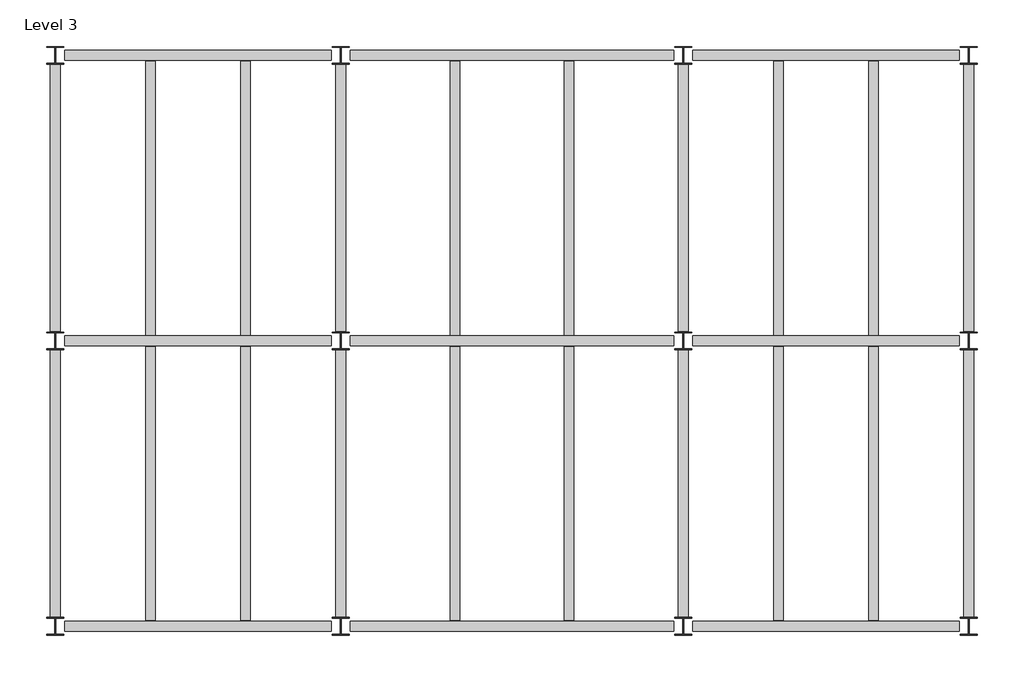
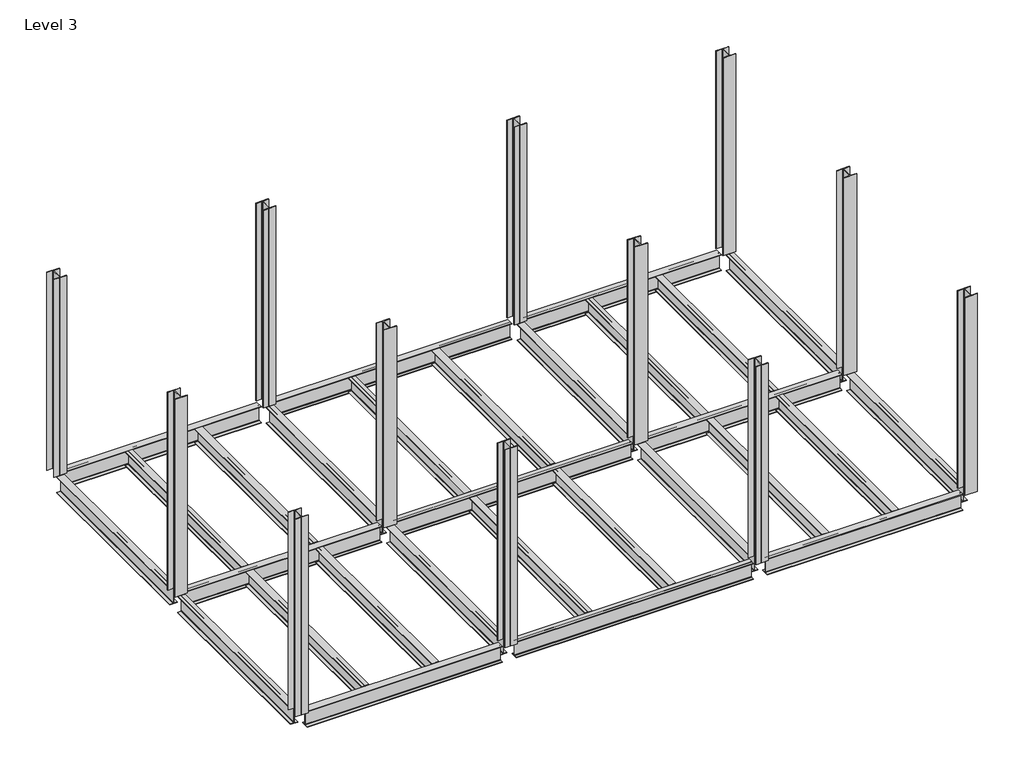
# One storey: 29 beams, 12 columns.
"""IFC4 building model written with IfcOpenShell, lengths in millimetres."""

import ifcopenshell
import ifcopenshell.guid

model = None  # the IFC model being written
_history = None  # IfcOwnerHistory: only IFC2X3 demands one
_inside = {}  # id of a spatial element -> (the spatial element, [elements in it])
_under = {}  # id of a project, library or spatial element -> (it, [spatial elements below it])
_declared = {}  # id of a project -> (the project, [libraries it declares])
_typed = {}  # id of a type object -> (the type object, [elements of that type])
_made_of = {}  # id of a material, layer set ... -> (it, [elements and type objects made of it])


def new_model(schema):
    """Start an empty IFC model of exactly this schema.

    Asked for "IFC4X3", IfcOpenShell would pick the latest addendum, in which some entities
    have other attributes; the version numbers below select the first issue.
    IFC2X3 requires an IfcOwnerHistory on every rooted entity: one is made here for all.
    """
    global model, _history
    if schema == "IFC4X3":
        model = ifcopenshell.file(schema_version=(4, 3, 0, 0))
    else:
        model = ifcopenshell.file(schema=schema)
    _inside.clear()
    _under.clear()
    _declared.clear()
    _typed.clear()
    _made_of.clear()
    _history = None
    if model.schema == "IFC2X3":
        org = make("IfcOrganization", Name="unknown")
        user = make(
            "IfcPersonAndOrganization",
            ThePerson=make("IfcPerson", FamilyName="unknown"),
            TheOrganization=org,
        )
        app = make(
            "IfcApplication",
            ApplicationDeveloper=org,
            Version="unknown",
            ApplicationFullName="unknown",
            ApplicationIdentifier="unknown",
        )
        _history = make(
            "IfcOwnerHistory",
            OwningUser=user,
            OwningApplication=app,
            ChangeAction="ADDED",
            CreationDate=0,
        )
    return model


def make(cls, **values):
    """One entity of the class cls with the attributes given. An attribute that is None is left unset."""
    return model.create_entity(
        cls, **{name: value for name, value in values.items() if value is not None}
    )


def rooted(cls, **values):
    """An entity with a GlobalId (a new one), such as an element, a storey or a relation."""
    return make(cls, GlobalId=ifcopenshell.guid.new(), OwnerHistory=_history, **values)


def si_unit(unit_type, name, prefix=None):
    """IfcSIUnit, for example si_unit("LENGTHUNIT", "METRE", prefix="MILLI")."""
    return make("IfcSIUnit", UnitType=unit_type, Prefix=prefix, Name=name)


def assignment(units):
    """IfcUnitAssignment: the units of a project."""
    return None if units is None else make("IfcUnitAssignment", Units=units)


def point(xyz):
    """IfcCartesianPoint."""
    return None if xyz is None else make("IfcCartesianPoint", Coordinates=xyz)


def direction(xyz):
    """IfcDirection."""
    return None if xyz is None else make("IfcDirection", DirectionRatios=xyz)


def frame(location, z_axis=None, x_axis=None):
    """IfcAxis2Placement3D, a coordinate frame: its origin and axes. An axis left out is left unset."""
    return make(
        "IfcAxis2Placement3D",
        Location=point(location),
        Axis=direction(z_axis),
        RefDirection=direction(x_axis),
    )


def frame_2d(location, x_axis=None):
    """IfcAxis2Placement2D, a coordinate frame in the plane: its origin and x axis."""
    return make(
        "IfcAxis2Placement2D", Location=point(location), RefDirection=direction(x_axis)
    )


def origin():
    """The frame at (0, 0, 0) with its axes left unset."""
    return frame((0.0, 0.0, 0.0))


def place(relative_to, where):
    """IfcLocalPlacement: puts the frame where relative to a parent placement (None: the world)."""
    return make(
        "IfcLocalPlacement", PlacementRelTo=relative_to, RelativePlacement=where
    )


def context(
    kind, dimensions, precision=None, world=None, true_north=None, identifier=None
):
    """IfcGeometricRepresentationContext, for example the 3D "Model" context."""
    return make(
        "IfcGeometricRepresentationContext",
        ContextIdentifier=identifier,
        ContextType=kind,
        CoordinateSpaceDimension=dimensions,
        Precision=precision,
        WorldCoordinateSystem=world,
        TrueNorth=true_north,
    )


def project(units=None, contexts=None):
    """IfcProject with its units and contexts."""
    return rooted(
        "IfcProject",
        Name="project",
        RepresentationContexts=contexts,
        UnitsInContext=assignment(units),
    )


def spatial(cls, under=None, at=None, **own):
    """A site, building, storey or space (cls), placed at a placement, below another one or the project."""
    s = rooted(cls, ObjectPlacement=at, **own)
    if under is not None:
        _under.setdefault(under.id(), (under, []))[1].append(s)
    return s


def polyline(points):
    """IfcPolyline through the points."""
    return make("IfcPolyline", Points=[point(p) for p in points])


def circle_curve(where, radius):
    """IfcCircle in the frame where."""
    return make("IfcCircle", Position=where, Radius=radius)


def trimmed(basis, trim1, trim2, sense, master):
    """IfcTrimmedCurve: the piece of a basis curve between two trims."""
    return make(
        "IfcTrimmedCurve",
        BasisCurve=basis,
        Trim1=trim1,
        Trim2=trim2,
        SenseAgreement=sense,
        MasterRepresentation=master,
    )


def segment(curve, same_sense, transition):
    """IfcCompositeCurveSegment."""
    return make(
        "IfcCompositeCurveSegment",
        Transition=transition,
        SameSense=same_sense,
        ParentCurve=curve,
    )


def composite_curve(segments, self_intersect=None):
    """IfcCompositeCurve: segments joined end to end."""
    return make("IfcCompositeCurve", Segments=segments, SelfIntersect=self_intersect)


def outline(outer, holes=None, kind="AREA"):
    """IfcArbitraryClosedProfileDef: a profile drawn as a closed curve; with holes, ...WithVoids."""
    if holes is None:
        return make("IfcArbitraryClosedProfileDef", ProfileType=kind, OuterCurve=outer)
    return make(
        "IfcArbitraryProfileDefWithVoids",
        ProfileType=kind,
        OuterCurve=outer,
        InnerCurves=holes,
    )


def extrude(swept, where, along, depth):
    """IfcExtrudedAreaSolid: the profile swept, set in the frame where, extruded along a direction by depth."""
    return make(
        "IfcExtrudedAreaSolid",
        SweptArea=swept,
        Position=where,
        ExtrudedDirection=direction(along),
        Depth=depth,
    )


def shape(context_of_items, identifier, shape_type, items):
    """IfcShapeRepresentation: the items that make up one representation, for example the "Body"."""
    return make(
        "IfcShapeRepresentation",
        ContextOfItems=context_of_items,
        RepresentationIdentifier=identifier,
        RepresentationType=shape_type,
        Items=items,
    )


def source(mapping_origin, context_of_items, identifier, shape_type, items):
    """IfcRepresentationMap: a shape defined once, which mapped items show again and again."""
    return make(
        "IfcRepresentationMap",
        MappingOrigin=mapping_origin,
        MappedRepresentation=shape(context_of_items, identifier, shape_type, items),
    )


def transform(
    local_origin,
    x_axis=None,
    y_axis=None,
    z_axis=None,
    scale=None,
    scale2=None,
    scale3=None,
    uniform=True,
):
    """IfcCartesianTransformationOperator3D, or its non-uniform kind. x_axis, y_axis, z_axis: its Axis1, 2, 3."""
    if uniform:
        return make(
            "IfcCartesianTransformationOperator3D",
            Axis1=direction(x_axis),
            Axis2=direction(y_axis),
            LocalOrigin=point(local_origin),
            Scale=scale,
            Axis3=direction(z_axis),
        )
    return make(
        "IfcCartesianTransformationOperator3DnonUniform",
        Axis1=direction(x_axis),
        Axis2=direction(y_axis),
        LocalOrigin=point(local_origin),
        Scale=scale,
        Axis3=direction(z_axis),
        Scale2=scale2,
        Scale3=scale3,
    )


def mapped(mapping_source, mapping_target):
    """IfcMappedItem: shows the shape of a source again, moved by a transform."""
    return make(
        "IfcMappedItem", MappingSource=mapping_source, MappingTarget=mapping_target
    )


def made_of(thing, what):
    """Note that an element or type object is made of a material, layer set ...; save() writes the relation."""
    if what is not None:
        _made_of.setdefault(what.id(), (what, []))[1].append(thing)
    return thing


def element(
    cls,
    number,
    at=None,
    inside=None,
    cuts=None,
    type_object=None,
    material=None,
    context=None,
    identifier="Body",
    shape_type=None,
    held_by="IfcProductDefinitionShape",
    body=None,
    shapes=None,
    **own,
):
    """One element of the class cls, such as IfcWall. Its Tag is "e" and its number.

    at: its placement. inside: the storey or other place that contains it. cuts: it is an
    opening in that element (IfcRelVoidsElement). A single representation is given by context,
    identifier, shape_type and body (its items); several are given by shapes. held_by: the class
    of the entity that holds the representations. save() writes the other relations.
    """
    e = rooted(cls, Tag="e%d" % number, ObjectPlacement=at, **own)
    if body is not None:
        shapes = [shape(context, identifier, shape_type, body)]
    if shapes is not None:
        e.Representation = make(held_by, Representations=shapes)
    if inside is not None:
        _inside.setdefault(inside.id(), (inside, []))[1].append(e)
    if cuts is not None:
        rooted(
            "IfcRelVoidsElement", RelatingBuildingElement=cuts, RelatedOpeningElement=e
        )
    if type_object is not None:
        _typed.setdefault(type_object.id(), (type_object, []))[1].append(e)
    return made_of(e, material)


def aggregate(whole, parts):
    """IfcRelAggregates: a whole, such as a stair, and the parts it consists of."""
    return rooted("IfcRelAggregates", RelatingObject=whole, RelatedObjects=parts)


def save(model, path):
    """Write the relations noted so far, then the file.

    IfcRelAggregates (storeys below a building ...), IfcRelContainedInSpatialStructure (elements
    in a storey), IfcRelDefinesByType, IfcRelAssociatesMaterial and IfcRelDeclares: one each for
    every whole, place, type object, material and project.
    """
    for whole, parts in _under.values():
        aggregate(whole, parts)
    for where, things in _inside.values():
        rooted(
            "IfcRelContainedInSpatialStructure",
            RelatedElements=things,
            RelatingStructure=where,
        )
    for kind, things in _typed.values():
        rooted("IfcRelDefinesByType", RelatedObjects=things, RelatingType=kind)
    for what, things in _made_of.values():
        rooted("IfcRelAssociatesMaterial", RelatedObjects=things, RelatingMaterial=what)
    for by, libraries in _declared.values():
        rooted("IfcRelDeclares", RelatingContext=by, RelatedDefinitions=libraries)
    model.write(path)


def ub_universal_beams_ub356x171x51_26e98692(model_context):
    return source(origin(), model_context, "Body", "SweptSolid", [
        extrude(outline(composite_curve([segment(polyline([(85.75, -166.0), (85.75, -177.5), (-85.75, -177.5), (-85.75, -166.0), (-13.9, -166.0)]), True, "CONTINUOUS"), segment(trimmed(circle_curve(frame_2d((-13.9, -155.8)), 10.2), [point((-13.9, -166.0))], [point((-3.7, -155.8))], True, "CARTESIAN"), True, "CONTINUOUS"), segment(polyline([(-3.7, -155.8), (-3.7, 155.8)]), True, "CONTINUOUS"), segment(trimmed(circle_curve(frame_2d((-13.9, 155.8)), 10.2), [point((-3.7, 155.8))], [point((-13.9, 166.0))], True, "CARTESIAN"), True, "CONTINUOUS"), segment(polyline([(-13.9, 166.0), (-85.75, 166.0), (-85.75, 177.5), (85.75, 177.5), (85.75, 166.0), (13.9, 166.0)]), True, "CONTINUOUS"), segment(trimmed(circle_curve(frame_2d((13.9, 155.8)), 10.2), [point((13.9, 166.0))], [point((3.7, 155.8))], True, "CARTESIAN"), True, "CONTINUOUS"), segment(polyline([(3.7, 155.8), (3.7, -155.8)]), True, "CONTINUOUS"), segment(trimmed(circle_curve(frame_2d((13.9, -155.8)), 10.2), [point((3.7, -155.8))], [point((13.9, -166.0))], True, "CARTESIAN"), True, "CONTINUOUS"), segment(polyline([(13.9, -166.0), (85.75, -166.0)]), True, "CONTINUOUS")], self_intersect=False)), frame((-2398.3, 0.0, 0.0), z_axis=(1.0, 0.0, 0.0), x_axis=(0.0, 1.0, 0.0)), (0.0, 0.0, 1.0), 4796.6),
    ])


def ub_universal_beams_ub406x178x60_425a89a6(model_context):
    return source(origin(), model_context, "Body", "SweptSolid", [
        extrude(outline(composite_curve([segment(polyline([(88.95, -190.4), (88.95, -203.2), (-88.95, -203.2), (-88.95, -190.4), (-14.15, -190.4)]), True, "CONTINUOUS"), segment(trimmed(circle_curve(frame_2d((-14.15, -180.2)), 10.2), [point((-14.15, -190.4))], [point((-3.95, -180.2))], True, "CARTESIAN"), True, "CONTINUOUS"), segment(polyline([(-3.95, -180.2), (-3.95, 180.2)]), True, "CONTINUOUS"), segment(trimmed(circle_curve(frame_2d((-14.15, 180.2)), 10.2), [point((-3.95, 180.2))], [point((-14.15, 190.4))], True, "CARTESIAN"), True, "CONTINUOUS"), segment(polyline([(-14.15, 190.4), (-88.95, 190.4), (-88.95, 203.2), (88.95, 203.2), (88.95, 190.4), (14.15, 190.4)]), True, "CONTINUOUS"), segment(trimmed(circle_curve(frame_2d((14.15, 180.2)), 10.2), [point((14.15, 190.4))], [point((3.95, 180.2))], True, "CARTESIAN"), True, "CONTINUOUS"), segment(polyline([(3.95, 180.2), (3.95, -180.2)]), True, "CONTINUOUS"), segment(trimmed(circle_curve(frame_2d((14.15, -180.2)), 10.2), [point((3.95, -180.2))], [point((14.15, -190.4))], True, "CARTESIAN"), True, "CONTINUOUS"), segment(polyline([(14.15, -190.4), (88.95, -190.4)]), True, "CONTINUOUS")], self_intersect=False)), frame((-2334.6, 0.0, 0.0), z_axis=(1.0, 0.0, 0.0), x_axis=(0.0, 1.0, 0.0)), (0.0, 0.0, 1.0), 4669.2),
    ])


def ub_universal_beams_ub406x178x60_ab0c7e2f(model_context):
    return source(origin(), model_context, "Body", "SweptSolid", [
        extrude(outline(composite_curve([segment(polyline([(88.95, -190.4), (88.95, -203.2), (-88.95, -203.2), (-88.95, -190.4), (-14.15, -190.4)]), True, "CONTINUOUS"), segment(trimmed(circle_curve(frame_2d((-14.15, -180.2)), 10.2), [point((-14.15, -190.4))], [point((-3.95, -180.2))], True, "CARTESIAN"), True, "CONTINUOUS"), segment(polyline([(-3.95, -180.2), (-3.95, 180.2)]), True, "CONTINUOUS"), segment(trimmed(circle_curve(frame_2d((-14.15, 180.2)), 10.2), [point((-3.95, 180.2))], [point((-14.15, 190.4))], True, "CARTESIAN"), True, "CONTINUOUS"), segment(polyline([(-14.15, 190.4), (-88.95, 190.4), (-88.95, 203.2), (88.95, 203.2), (88.95, 190.4), (14.15, 190.4)]), True, "CONTINUOUS"), segment(trimmed(circle_curve(frame_2d((14.15, 180.2)), 10.2), [point((14.15, 190.4))], [point((3.95, 180.2))], True, "CARTESIAN"), True, "CONTINUOUS"), segment(polyline([(3.95, 180.2), (3.95, -180.2)]), True, "CONTINUOUS"), segment(trimmed(circle_curve(frame_2d((14.15, -180.2)), 10.2), [point((3.95, -180.2))], [point((14.15, -190.4))], True, "CARTESIAN"), True, "CONTINUOUS"), segment(polyline([(14.15, -190.4), (88.95, -190.4)]), True, "CONTINUOUS")], self_intersect=False)), frame((-2834.6, 0.0, 0.0), z_axis=(1.0, 0.0, 0.0), x_axis=(0.0, 1.0, 0.0)), (0.0, 0.0, 1.0), 5669.2),
    ])


def ub_universal_beams_ub406x178x60_873acc54(model_context):
    return source(origin(), model_context, "Body", "SweptSolid", [
        extrude(outline(composite_curve([segment(polyline([(88.95, -190.4), (88.95, -203.2), (-88.95, -203.2), (-88.95, -190.4), (-14.15, -190.4)]), True, "CONTINUOUS"), segment(trimmed(circle_curve(frame_2d((-14.15, -180.2)), 10.2), [point((-14.15, -190.4))], [point((-3.95, -180.2))], True, "CARTESIAN"), True, "CONTINUOUS"), segment(polyline([(-3.95, -180.2), (-3.95, 180.2)]), True, "CONTINUOUS"), segment(trimmed(circle_curve(frame_2d((-14.15, 180.2)), 10.2), [point((-3.95, 180.2))], [point((-14.15, 190.4))], True, "CARTESIAN"), True, "CONTINUOUS"), segment(polyline([(-14.15, 190.4), (-88.95, 190.4), (-88.95, 203.2), (88.95, 203.2), (88.95, 190.4), (14.15, 190.4)]), True, "CONTINUOUS"), segment(trimmed(circle_curve(frame_2d((14.15, 180.2)), 10.2), [point((14.15, 190.4))], [point((3.95, 180.2))], True, "CARTESIAN"), True, "CONTINUOUS"), segment(polyline([(3.95, 180.2), (3.95, -180.2)]), True, "CONTINUOUS"), segment(trimmed(circle_curve(frame_2d((14.15, -180.2)), 10.2), [point((3.95, -180.2))], [point((14.15, -190.4))], True, "CARTESIAN"), True, "CONTINUOUS"), segment(polyline([(14.15, -190.4), (88.95, -190.4)]), True, "CONTINUOUS")], self_intersect=False)), frame((-2333.3, 0.0, 0.0), z_axis=(1.0, 0.0, 0.0), x_axis=(0.0, 1.0, 0.0)), (0.0, 0.0, 1.0), 4666.6),
    ])


model = new_model("IFC4")

# Units and contexts
model_context = context("Model", 3, world=origin())
ifc_project = project(units=[si_unit("LENGTHUNIT", "METRE", prefix="MILLI")], contexts=[model_context])

# Site, building, storey
site = spatial("IfcSite", under=ifc_project)
building = spatial("IfcBuilding", under=site)
storey = spatial("IfcBuildingStorey", under=building, Name="Level 3", Elevation=4000.0)

# Beams
placement = place(None, origin())
ub_universal_beams_ub356x171x51_shape = ub_universal_beams_ub356x171x51_26e98692(model_context)
element("IfcBeam", 1, ObjectType="UB-Universal Beams : UB356x171x51", at=placement, inside=storey, context=model_context, shape_type="MappedRepresentation", body=[
    mapped(ub_universal_beams_ub356x171x51_shape, transform((1666.6666667, 2500.0, 3822.5), x_axis=(0.0, 1.0, 0.0), y_axis=(-1.0, 0.0, 0.0), z_axis=(0.0, 0.0, 1.0))),
])
element("IfcBeam", 2, ObjectType="UB-Universal Beams : UB356x171x51", at=placement, inside=storey, context=model_context, shape_type="MappedRepresentation", body=[
    mapped(ub_universal_beams_ub356x171x51_shape, transform((3333.3333333, 2500.0, 3822.5), x_axis=(0.0, 1.0, 0.0), y_axis=(-1.0, 0.0, 0.0), z_axis=(0.0, 0.0, 1.0))),
])
element("IfcBeam", 3, ObjectType="UB-Universal Beams : UB356x171x51", at=placement, inside=storey, context=model_context, shape_type="MappedRepresentation", body=[
    mapped(ub_universal_beams_ub356x171x51_shape, transform((7000.0, 2500.0, 3822.5), x_axis=(0.0, 1.0, 0.0), y_axis=(-1.0, 0.0, 0.0), z_axis=(0.0, 0.0, 1.0))),
])
element("IfcBeam", 4, ObjectType="UB-Universal Beams : UB356x171x51", at=placement, inside=storey, context=model_context, shape_type="MappedRepresentation", body=[
    mapped(ub_universal_beams_ub356x171x51_shape, transform((9000.0, 2500.0, 3822.5), x_axis=(0.0, 1.0, 0.0), y_axis=(-1.0, 0.0, 0.0), z_axis=(0.0, 0.0, 1.0))),
])
element("IfcBeam", 5, ObjectType="UB-Universal Beams : UB356x171x51", at=placement, inside=storey, context=model_context, shape_type="MappedRepresentation", body=[
    mapped(ub_universal_beams_ub356x171x51_shape, transform((12666.6666667, 2500.0, 3822.5), x_axis=(0.0, 1.0, 0.0), y_axis=(-1.0, 0.0, 0.0), z_axis=(0.0, 0.0, 1.0))),
])
element("IfcBeam", 6, ObjectType="UB-Universal Beams : UB356x171x51", at=placement, inside=storey, context=model_context, shape_type="MappedRepresentation", body=[
    mapped(ub_universal_beams_ub356x171x51_shape, transform((14333.3333333, 2500.0, 3822.5), x_axis=(0.0, 1.0, 0.0), y_axis=(-1.0, 0.0, 0.0), z_axis=(0.0, 0.0, 1.0))),
])
element("IfcBeam", 7, ObjectType="UB-Universal Beams : UB356x171x51", at=placement, inside=storey, context=model_context, shape_type="MappedRepresentation", body=[
    mapped(ub_universal_beams_ub356x171x51_shape, transform((1666.6666667, 7500.0, 3822.5), x_axis=(0.0, 1.0, 0.0), y_axis=(-1.0, 0.0, 0.0), z_axis=(0.0, 0.0, 1.0))),
])
element("IfcBeam", 8, ObjectType="UB-Universal Beams : UB356x171x51", at=placement, inside=storey, context=model_context, shape_type="MappedRepresentation", body=[
    mapped(ub_universal_beams_ub356x171x51_shape, transform((3333.3333333, 7500.0, 3822.5), x_axis=(0.0, 1.0, 0.0), y_axis=(-1.0, 0.0, 0.0), z_axis=(0.0, 0.0, 1.0))),
])
element("IfcBeam", 9, ObjectType="UB-Universal Beams : UB356x171x51", at=placement, inside=storey, context=model_context, shape_type="MappedRepresentation", body=[
    mapped(ub_universal_beams_ub356x171x51_shape, transform((7000.0, 7500.0, 3822.5), x_axis=(0.0, 1.0, 0.0), y_axis=(-1.0, 0.0, 0.0), z_axis=(0.0, 0.0, 1.0))),
])
element("IfcBeam", 10, ObjectType="UB-Universal Beams : UB356x171x51", at=placement, inside=storey, context=model_context, shape_type="MappedRepresentation", body=[
    mapped(ub_universal_beams_ub356x171x51_shape, transform((9000.0, 7500.0, 3822.5), x_axis=(0.0, 1.0, 0.0), y_axis=(-1.0, 0.0, 0.0), z_axis=(0.0, 0.0, 1.0))),
])
element("IfcBeam", 11, ObjectType="UB-Universal Beams : UB356x171x51", at=placement, inside=storey, context=model_context, shape_type="MappedRepresentation", body=[
    mapped(ub_universal_beams_ub356x171x51_shape, transform((12666.6666667, 7500.0, 3822.5), x_axis=(0.0, 1.0, 0.0), y_axis=(-1.0, 0.0, 0.0), z_axis=(0.0, 0.0, 1.0))),
])
element("IfcBeam", 12, ObjectType="UB-Universal Beams : UB356x171x51", at=placement, inside=storey, context=model_context, shape_type="MappedRepresentation", body=[
    mapped(ub_universal_beams_ub356x171x51_shape, transform((14333.3333333, 7500.0, 3822.5), x_axis=(0.0, 1.0, 0.0), y_axis=(-1.0, 0.0, 0.0), z_axis=(0.0, 0.0, 1.0))),
])
ub_universal_beams_ub406x178x60_shape = ub_universal_beams_ub406x178x60_425a89a6(model_context)
element("IfcBeam", 13, ObjectType="UB-Universal Beams : UB406x178x60", at=placement, inside=storey, context=model_context, shape_type="MappedRepresentation", body=[
    mapped(ub_universal_beams_ub406x178x60_shape, transform((2500.0, 0.0, 3796.8), x_axis=(1.0, 0.0, 0.0), y_axis=(0.0, 1.0, 0.0), z_axis=(0.0, 0.0, 1.0))),
])
element("IfcBeam", 14, ObjectType="UB-Universal Beams : UB406x178x60", at=placement, inside=storey, context=model_context, shape_type="MappedRepresentation", body=[
    mapped(ub_universal_beams_ub406x178x60_shape, transform((13500.0, 0.0, 3796.8), x_axis=(1.0, 0.0, 0.0), y_axis=(0.0, 1.0, 0.0), z_axis=(0.0, 0.0, 1.0))),
])
element("IfcBeam", 15, ObjectType="UB-Universal Beams : UB406x178x60", at=placement, inside=storey, context=model_context, shape_type="MappedRepresentation", body=[
    mapped(ub_universal_beams_ub406x178x60_shape, transform((2500.0, 5000.0, 3796.8), x_axis=(1.0, 0.0, 0.0), y_axis=(0.0, 1.0, 0.0), z_axis=(0.0, 0.0, 1.0))),
])
element("IfcBeam", 16, ObjectType="UB-Universal Beams : UB406x178x60", at=placement, inside=storey, context=model_context, shape_type="MappedRepresentation", body=[
    mapped(ub_universal_beams_ub406x178x60_shape, transform((13500.0, 5000.0, 3796.8), x_axis=(1.0, 0.0, 0.0), y_axis=(0.0, 1.0, 0.0), z_axis=(0.0, 0.0, 1.0))),
])
element("IfcBeam", 17, ObjectType="UB-Universal Beams : UB406x178x60", at=placement, inside=storey, context=model_context, shape_type="MappedRepresentation", body=[
    mapped(ub_universal_beams_ub406x178x60_shape, transform((2500.0, 10000.0, 3796.8), x_axis=(1.0, 0.0, 0.0), y_axis=(0.0, 1.0, 0.0), z_axis=(0.0, 0.0, 1.0))),
])
element("IfcBeam", 18, ObjectType="UB-Universal Beams : UB406x178x60", at=placement, inside=storey, context=model_context, shape_type="MappedRepresentation", body=[
    mapped(ub_universal_beams_ub406x178x60_shape, transform((13500.0, 10000.0, 3796.8), x_axis=(1.0, 0.0, 0.0), y_axis=(0.0, 1.0, 0.0), z_axis=(0.0, 0.0, 1.0))),
])
ub_universal_beams_ub406x178x60_2_shape = ub_universal_beams_ub406x178x60_ab0c7e2f(model_context)
element("IfcBeam", 19, ObjectType="UB-Universal Beams : UB406x178x60", at=placement, inside=storey, context=model_context, shape_type="MappedRepresentation", body=[
    mapped(ub_universal_beams_ub406x178x60_2_shape, transform((8000.0, 0.0, 3796.8), x_axis=(1.0, 0.0, 0.0), y_axis=(0.0, 1.0, 0.0), z_axis=(0.0, 0.0, 1.0))),
])
element("IfcBeam", 20, ObjectType="UB-Universal Beams : UB406x178x60", at=placement, inside=storey, context=model_context, shape_type="MappedRepresentation", body=[
    mapped(ub_universal_beams_ub406x178x60_2_shape, transform((8000.0, 5000.0, 3796.8), x_axis=(1.0, 0.0, 0.0), y_axis=(0.0, 1.0, 0.0), z_axis=(0.0, 0.0, 1.0))),
])
element("IfcBeam", 21, ObjectType="UB-Universal Beams : UB406x178x60", at=placement, inside=storey, context=model_context, shape_type="MappedRepresentation", body=[
    mapped(ub_universal_beams_ub406x178x60_2_shape, transform((8000.0, 10000.0, 3796.8), x_axis=(1.0, 0.0, 0.0), y_axis=(0.0, 1.0, 0.0), z_axis=(0.0, 0.0, 1.0))),
])
ub_universal_beams_ub406x178x60_3_shape = ub_universal_beams_ub406x178x60_873acc54(model_context)
element("IfcBeam", 22, ObjectType="UB-Universal Beams : UB406x178x60", at=placement, inside=storey, context=model_context, shape_type="MappedRepresentation", body=[
    mapped(ub_universal_beams_ub406x178x60_3_shape, transform((0.0, 2500.0, 3796.8), x_axis=(0.0, 1.0, 0.0), y_axis=(-1.0, 0.0, 0.0), z_axis=(0.0, 0.0, 1.0))),
])
element("IfcBeam", 23, ObjectType="UB-Universal Beams : UB406x178x60", at=placement, inside=storey, context=model_context, shape_type="MappedRepresentation", body=[
    mapped(ub_universal_beams_ub406x178x60_3_shape, transform((0.0, 7500.0, 3796.8), x_axis=(0.0, 1.0, 0.0), y_axis=(-1.0, 0.0, 0.0), z_axis=(0.0, 0.0, 1.0))),
])
element("IfcBeam", 24, ObjectType="UB-Universal Beams : UB406x178x60", at=placement, inside=storey, context=model_context, shape_type="MappedRepresentation", body=[
    mapped(ub_universal_beams_ub406x178x60_3_shape, transform((5000.0, 2500.0, 3796.8), x_axis=(0.0, 1.0, 0.0), y_axis=(-1.0, 0.0, 0.0), z_axis=(0.0, 0.0, 1.0))),
])
element("IfcBeam", 25, ObjectType="UB-Universal Beams : UB406x178x60", at=placement, inside=storey, context=model_context, shape_type="MappedRepresentation", body=[
    mapped(ub_universal_beams_ub406x178x60_3_shape, transform((5000.0, 7500.0, 3796.8), x_axis=(0.0, 1.0, 0.0), y_axis=(-1.0, 0.0, 0.0), z_axis=(0.0, 0.0, 1.0))),
])
element("IfcBeam", 26, ObjectType="UB-Universal Beams : UB406x178x60", at=placement, inside=storey, context=model_context, shape_type="MappedRepresentation", body=[
    mapped(ub_universal_beams_ub406x178x60_3_shape, transform((11000.0, 2500.0, 3796.8), x_axis=(0.0, 1.0, 0.0), y_axis=(-1.0, 0.0, 0.0), z_axis=(0.0, 0.0, 1.0))),
])
element("IfcBeam", 27, ObjectType="UB-Universal Beams : UB406x178x60", at=placement, inside=storey, context=model_context, shape_type="MappedRepresentation", body=[
    mapped(ub_universal_beams_ub406x178x60_3_shape, transform((11000.0, 7500.0, 3796.8), x_axis=(0.0, 1.0, 0.0), y_axis=(-1.0, 0.0, 0.0), z_axis=(0.0, 0.0, 1.0))),
])
element("IfcBeam", 28, ObjectType="UB-Universal Beams : UB406x178x60", at=placement, inside=storey, context=model_context, shape_type="MappedRepresentation", body=[
    mapped(ub_universal_beams_ub406x178x60_3_shape, transform((16000.0, 2500.0, 3796.8), x_axis=(0.0, 1.0, 0.0), y_axis=(-1.0, 0.0, 0.0), z_axis=(0.0, 0.0, 1.0))),
])
element("IfcBeam", 29, ObjectType="UB-Universal Beams : UB406x178x60", at=placement, inside=storey, context=model_context, shape_type="MappedRepresentation", body=[
    mapped(ub_universal_beams_ub406x178x60_3_shape, transform((16000.0, 7500.0, 3796.8), x_axis=(0.0, 1.0, 0.0), y_axis=(-1.0, 0.0, 0.0), z_axis=(0.0, 0.0, 1.0))),
])

# Columns
element("IfcColumn", 30, ObjectType="UC-Universal Columns-Column : UC305x305x97", at=placement, inside=storey, context=model_context, shape_type="SweptSolid", body=[
    extrude(outline(composite_curve([segment(polyline([(152.65, 153.95), (152.65, 138.55), (20.15, 138.55)]), True, "CONTINUOUS"), segment(trimmed(circle_curve(frame_2d((20.15, 123.35)), 15.2), [point((20.15, 138.55))], [point((4.95, 123.35))], True, "CARTESIAN"), True, "CONTINUOUS"), segment(polyline([(4.95, 123.35), (4.95, -123.35)]), True, "CONTINUOUS"), segment(trimmed(circle_curve(frame_2d((20.15, -123.35)), 15.2), [point((4.95, -123.35))], [point((20.15, -138.55))], True, "CARTESIAN"), True, "CONTINUOUS"), segment(polyline([(20.15, -138.55), (152.65, -138.55), (152.65, -153.95), (-152.65, -153.95), (-152.65, -138.55), (-20.15, -138.55)]), True, "CONTINUOUS"), segment(trimmed(circle_curve(frame_2d((-20.15, -123.35)), 15.2), [point((-20.15, -138.55))], [point((-4.95, -123.35))], True, "CARTESIAN"), True, "CONTINUOUS"), segment(polyline([(-4.95, -123.35), (-4.95, 123.35)]), True, "CONTINUOUS"), segment(trimmed(circle_curve(frame_2d((-20.15, 123.35)), 15.2), [point((-4.95, 123.35))], [point((-20.15, 138.55))], True, "CARTESIAN"), True, "CONTINUOUS"), segment(polyline([(-20.15, 138.55), (-152.65, 138.55), (-152.65, 153.95), (152.65, 153.95)]), True, "CONTINUOUS")], self_intersect=False)), frame((0.0, 0.0, 4000.0), z_axis=(0.0, 0.0, 1.0), x_axis=(1.0, 0.0, 0.0)), (0.0, 0.0, 1.0), 5000.0),
])
element("IfcColumn", 31, ObjectType="UC-Universal Columns-Column : UC305x305x97", at=placement, inside=storey, context=model_context, shape_type="SweptSolid", body=[
    extrude(outline(composite_curve([segment(polyline([(5152.65, 153.95), (5152.65, 138.55), (5020.15, 138.55)]), True, "CONTINUOUS"), segment(trimmed(circle_curve(frame_2d((5020.15, 123.35)), 15.2), [point((5020.15, 138.55))], [point((5004.95, 123.35))], True, "CARTESIAN"), True, "CONTINUOUS"), segment(polyline([(5004.95, 123.35), (5004.95, -123.35)]), True, "CONTINUOUS"), segment(trimmed(circle_curve(frame_2d((5020.15, -123.35)), 15.2), [point((5004.95, -123.35))], [point((5020.15, -138.55))], True, "CARTESIAN"), True, "CONTINUOUS"), segment(polyline([(5020.15, -138.55), (5152.65, -138.55), (5152.65, -153.95), (4847.35, -153.95), (4847.35, -138.55), (4979.85, -138.55)]), True, "CONTINUOUS"), segment(trimmed(circle_curve(frame_2d((4979.85, -123.35)), 15.2), [point((4979.85, -138.55))], [point((4995.05, -123.35))], True, "CARTESIAN"), True, "CONTINUOUS"), segment(polyline([(4995.05, -123.35), (4995.05, 123.35)]), True, "CONTINUOUS"), segment(trimmed(circle_curve(frame_2d((4979.85, 123.35)), 15.2), [point((4995.05, 123.35))], [point((4979.85, 138.55))], True, "CARTESIAN"), True, "CONTINUOUS"), segment(polyline([(4979.85, 138.55), (4847.35, 138.55), (4847.35, 153.95), (5152.65, 153.95)]), True, "CONTINUOUS")], self_intersect=False)), frame((0.0, 0.0, 4000.0), z_axis=(0.0, 0.0, 1.0), x_axis=(1.0, 0.0, 0.0)), (0.0, 0.0, 1.0), 5000.0),
])
element("IfcColumn", 32, ObjectType="UC-Universal Columns-Column : UC305x305x97", at=placement, inside=storey, context=model_context, shape_type="SweptSolid", body=[
    extrude(outline(composite_curve([segment(polyline([(11152.65, 153.95), (11152.65, 138.55), (11020.15, 138.55)]), True, "CONTINUOUS"), segment(trimmed(circle_curve(frame_2d((11020.15, 123.35)), 15.2), [point((11020.15, 138.55))], [point((11004.95, 123.35))], True, "CARTESIAN"), True, "CONTINUOUS"), segment(polyline([(11004.95, 123.35), (11004.95, -123.35)]), True, "CONTINUOUS"), segment(trimmed(circle_curve(frame_2d((11020.15, -123.35)), 15.2), [point((11004.95, -123.35))], [point((11020.15, -138.55))], True, "CARTESIAN"), True, "CONTINUOUS"), segment(polyline([(11020.15, -138.55), (11152.65, -138.55), (11152.65, -153.95), (10847.35, -153.95), (10847.35, -138.55), (10979.85, -138.55)]), True, "CONTINUOUS"), segment(trimmed(circle_curve(frame_2d((10979.85, -123.35)), 15.2), [point((10979.85, -138.55))], [point((10995.05, -123.35))], True, "CARTESIAN"), True, "CONTINUOUS"), segment(polyline([(10995.05, -123.35), (10995.05, 123.35)]), True, "CONTINUOUS"), segment(trimmed(circle_curve(frame_2d((10979.85, 123.35)), 15.2), [point((10995.05, 123.35))], [point((10979.85, 138.55))], True, "CARTESIAN"), True, "CONTINUOUS"), segment(polyline([(10979.85, 138.55), (10847.35, 138.55), (10847.35, 153.95), (11152.65, 153.95)]), True, "CONTINUOUS")], self_intersect=False)), frame((0.0, 0.0, 4000.0), z_axis=(0.0, 0.0, 1.0), x_axis=(1.0, 0.0, 0.0)), (0.0, 0.0, 1.0), 5000.0),
])
element("IfcColumn", 33, ObjectType="UC-Universal Columns-Column : UC305x305x97", at=placement, inside=storey, context=model_context, shape_type="SweptSolid", body=[
    extrude(outline(composite_curve([segment(polyline([(16152.65, 153.95), (16152.65, 138.55), (16020.15, 138.55)]), True, "CONTINUOUS"), segment(trimmed(circle_curve(frame_2d((16020.15, 123.35)), 15.2), [point((16020.15, 138.55))], [point((16004.95, 123.35))], True, "CARTESIAN"), True, "CONTINUOUS"), segment(polyline([(16004.95, 123.35), (16004.95, -123.35)]), True, "CONTINUOUS"), segment(trimmed(circle_curve(frame_2d((16020.15, -123.35)), 15.2), [point((16004.95, -123.35))], [point((16020.15, -138.55))], True, "CARTESIAN"), True, "CONTINUOUS"), segment(polyline([(16020.15, -138.55), (16152.65, -138.55), (16152.65, -153.95), (15847.35, -153.95), (15847.35, -138.55), (15979.85, -138.55)]), True, "CONTINUOUS"), segment(trimmed(circle_curve(frame_2d((15979.85, -123.35)), 15.2), [point((15979.85, -138.55))], [point((15995.05, -123.35))], True, "CARTESIAN"), True, "CONTINUOUS"), segment(polyline([(15995.05, -123.35), (15995.05, 123.35)]), True, "CONTINUOUS"), segment(trimmed(circle_curve(frame_2d((15979.85, 123.35)), 15.2), [point((15995.05, 123.35))], [point((15979.85, 138.55))], True, "CARTESIAN"), True, "CONTINUOUS"), segment(polyline([(15979.85, 138.55), (15847.35, 138.55), (15847.35, 153.95), (16152.65, 153.95)]), True, "CONTINUOUS")], self_intersect=False)), frame((0.0, 0.0, 4000.0), z_axis=(0.0, 0.0, 1.0), x_axis=(1.0, 0.0, 0.0)), (0.0, 0.0, 1.0), 5000.0),
])
element("IfcColumn", 34, ObjectType="UC-Universal Columns-Column : UC305x305x97", at=placement, inside=storey, context=model_context, shape_type="SweptSolid", body=[
    extrude(outline(composite_curve([segment(polyline([(152.65, 5153.95), (152.65, 5138.55), (20.15, 5138.55)]), True, "CONTINUOUS"), segment(trimmed(circle_curve(frame_2d((20.15, 5123.35)), 15.2), [point((20.15, 5138.55))], [point((4.95, 5123.35))], True, "CARTESIAN"), True, "CONTINUOUS"), segment(polyline([(4.95, 5123.35), (4.95, 4876.65)]), True, "CONTINUOUS"), segment(trimmed(circle_curve(frame_2d((20.15, 4876.65)), 15.2), [point((4.95, 4876.65))], [point((20.15, 4861.45))], True, "CARTESIAN"), True, "CONTINUOUS"), segment(polyline([(20.15, 4861.45), (152.65, 4861.45), (152.65, 4846.05), (-152.65, 4846.05), (-152.65, 4861.45), (-20.15, 4861.45)]), True, "CONTINUOUS"), segment(trimmed(circle_curve(frame_2d((-20.15, 4876.65)), 15.2), [point((-20.15, 4861.45))], [point((-4.95, 4876.65))], True, "CARTESIAN"), True, "CONTINUOUS"), segment(polyline([(-4.95, 4876.65), (-4.95, 5123.35)]), True, "CONTINUOUS"), segment(trimmed(circle_curve(frame_2d((-20.15, 5123.35)), 15.2), [point((-4.95, 5123.35))], [point((-20.15, 5138.55))], True, "CARTESIAN"), True, "CONTINUOUS"), segment(polyline([(-20.15, 5138.55), (-152.65, 5138.55), (-152.65, 5153.95), (152.65, 5153.95)]), True, "CONTINUOUS")], self_intersect=False)), frame((0.0, 0.0, 4000.0), z_axis=(0.0, 0.0, 1.0), x_axis=(1.0, 0.0, 0.0)), (0.0, 0.0, 1.0), 5000.0),
])
element("IfcColumn", 35, ObjectType="UC-Universal Columns-Column : UC305x305x97", at=placement, inside=storey, context=model_context, shape_type="SweptSolid", body=[
    extrude(outline(composite_curve([segment(polyline([(5152.65, 5153.95), (5152.65, 5138.55), (5020.15, 5138.55)]), True, "CONTINUOUS"), segment(trimmed(circle_curve(frame_2d((5020.15, 5123.35)), 15.2), [point((5020.15, 5138.55))], [point((5004.95, 5123.35))], True, "CARTESIAN"), True, "CONTINUOUS"), segment(polyline([(5004.95, 5123.35), (5004.95, 4876.65)]), True, "CONTINUOUS"), segment(trimmed(circle_curve(frame_2d((5020.15, 4876.65)), 15.2), [point((5004.95, 4876.65))], [point((5020.15, 4861.45))], True, "CARTESIAN"), True, "CONTINUOUS"), segment(polyline([(5020.15, 4861.45), (5152.65, 4861.45), (5152.65, 4846.05), (4847.35, 4846.05), (4847.35, 4861.45), (4979.85, 4861.45)]), True, "CONTINUOUS"), segment(trimmed(circle_curve(frame_2d((4979.85, 4876.65)), 15.2), [point((4979.85, 4861.45))], [point((4995.05, 4876.65))], True, "CARTESIAN"), True, "CONTINUOUS"), segment(polyline([(4995.05, 4876.65), (4995.05, 5123.35)]), True, "CONTINUOUS"), segment(trimmed(circle_curve(frame_2d((4979.85, 5123.35)), 15.2), [point((4995.05, 5123.35))], [point((4979.85, 5138.55))], True, "CARTESIAN"), True, "CONTINUOUS"), segment(polyline([(4979.85, 5138.55), (4847.35, 5138.55), (4847.35, 5153.95), (5152.65, 5153.95)]), True, "CONTINUOUS")], self_intersect=False)), frame((0.0, 0.0, 4000.0), z_axis=(0.0, 0.0, 1.0), x_axis=(1.0, 0.0, 0.0)), (0.0, 0.0, 1.0), 5000.0),
])
element("IfcColumn", 36, ObjectType="UC-Universal Columns-Column : UC305x305x97", at=placement, inside=storey, context=model_context, shape_type="SweptSolid", body=[
    extrude(outline(composite_curve([segment(polyline([(11152.65, 5153.95), (11152.65, 5138.55), (11020.15, 5138.55)]), True, "CONTINUOUS"), segment(trimmed(circle_curve(frame_2d((11020.15, 5123.35)), 15.2), [point((11020.15, 5138.55))], [point((11004.95, 5123.35))], True, "CARTESIAN"), True, "CONTINUOUS"), segment(polyline([(11004.95, 5123.35), (11004.95, 4876.65)]), True, "CONTINUOUS"), segment(trimmed(circle_curve(frame_2d((11020.15, 4876.65)), 15.2), [point((11004.95, 4876.65))], [point((11020.15, 4861.45))], True, "CARTESIAN"), True, "CONTINUOUS"), segment(polyline([(11020.15, 4861.45), (11152.65, 4861.45), (11152.65, 4846.05), (10847.35, 4846.05), (10847.35, 4861.45), (10979.85, 4861.45)]), True, "CONTINUOUS"), segment(trimmed(circle_curve(frame_2d((10979.85, 4876.65)), 15.2), [point((10979.85, 4861.45))], [point((10995.05, 4876.65))], True, "CARTESIAN"), True, "CONTINUOUS"), segment(polyline([(10995.05, 4876.65), (10995.05, 5123.35)]), True, "CONTINUOUS"), segment(trimmed(circle_curve(frame_2d((10979.85, 5123.35)), 15.2), [point((10995.05, 5123.35))], [point((10979.85, 5138.55))], True, "CARTESIAN"), True, "CONTINUOUS"), segment(polyline([(10979.85, 5138.55), (10847.35, 5138.55), (10847.35, 5153.95), (11152.65, 5153.95)]), True, "CONTINUOUS")], self_intersect=False)), frame((0.0, 0.0, 4000.0), z_axis=(0.0, 0.0, 1.0), x_axis=(1.0, 0.0, 0.0)), (0.0, 0.0, 1.0), 5000.0),
])
element("IfcColumn", 37, ObjectType="UC-Universal Columns-Column : UC305x305x97", at=placement, inside=storey, context=model_context, shape_type="SweptSolid", body=[
    extrude(outline(composite_curve([segment(polyline([(16152.65, 5153.95), (16152.65, 5138.55), (16020.15, 5138.55)]), True, "CONTINUOUS"), segment(trimmed(circle_curve(frame_2d((16020.15, 5123.35)), 15.2), [point((16020.15, 5138.55))], [point((16004.95, 5123.35))], True, "CARTESIAN"), True, "CONTINUOUS"), segment(polyline([(16004.95, 5123.35), (16004.95, 4876.65)]), True, "CONTINUOUS"), segment(trimmed(circle_curve(frame_2d((16020.15, 4876.65)), 15.2), [point((16004.95, 4876.65))], [point((16020.15, 4861.45))], True, "CARTESIAN"), True, "CONTINUOUS"), segment(polyline([(16020.15, 4861.45), (16152.65, 4861.45), (16152.65, 4846.05), (15847.35, 4846.05), (15847.35, 4861.45), (15979.85, 4861.45)]), True, "CONTINUOUS"), segment(trimmed(circle_curve(frame_2d((15979.85, 4876.65)), 15.2), [point((15979.85, 4861.45))], [point((15995.05, 4876.65))], True, "CARTESIAN"), True, "CONTINUOUS"), segment(polyline([(15995.05, 4876.65), (15995.05, 5123.35)]), True, "CONTINUOUS"), segment(trimmed(circle_curve(frame_2d((15979.85, 5123.35)), 15.2), [point((15995.05, 5123.35))], [point((15979.85, 5138.55))], True, "CARTESIAN"), True, "CONTINUOUS"), segment(polyline([(15979.85, 5138.55), (15847.35, 5138.55), (15847.35, 5153.95), (16152.65, 5153.95)]), True, "CONTINUOUS")], self_intersect=False)), frame((0.0, 0.0, 4000.0), z_axis=(0.0, 0.0, 1.0), x_axis=(1.0, 0.0, 0.0)), (0.0, 0.0, 1.0), 5000.0),
])
element("IfcColumn", 38, ObjectType="UC-Universal Columns-Column : UC305x305x97", at=placement, inside=storey, context=model_context, shape_type="SweptSolid", body=[
    extrude(outline(composite_curve([segment(polyline([(152.65, 10153.95), (152.65, 10138.55), (20.15, 10138.55)]), True, "CONTINUOUS"), segment(trimmed(circle_curve(frame_2d((20.15, 10123.35)), 15.2), [point((20.15, 10138.55))], [point((4.95, 10123.35))], True, "CARTESIAN"), True, "CONTINUOUS"), segment(polyline([(4.95, 10123.35), (4.95, 9876.65)]), True, "CONTINUOUS"), segment(trimmed(circle_curve(frame_2d((20.15, 9876.65)), 15.2), [point((4.95, 9876.65))], [point((20.15, 9861.45))], True, "CARTESIAN"), True, "CONTINUOUS"), segment(polyline([(20.15, 9861.45), (152.65, 9861.45), (152.65, 9846.05), (-152.65, 9846.05), (-152.65, 9861.45), (-20.15, 9861.45)]), True, "CONTINUOUS"), segment(trimmed(circle_curve(frame_2d((-20.15, 9876.65)), 15.2), [point((-20.15, 9861.45))], [point((-4.95, 9876.65))], True, "CARTESIAN"), True, "CONTINUOUS"), segment(polyline([(-4.95, 9876.65), (-4.95, 10123.35)]), True, "CONTINUOUS"), segment(trimmed(circle_curve(frame_2d((-20.15, 10123.35)), 15.2), [point((-4.95, 10123.35))], [point((-20.15, 10138.55))], True, "CARTESIAN"), True, "CONTINUOUS"), segment(polyline([(-20.15, 10138.55), (-152.65, 10138.55), (-152.65, 10153.95), (152.65, 10153.95)]), True, "CONTINUOUS")], self_intersect=False)), frame((0.0, 0.0, 4000.0), z_axis=(0.0, 0.0, 1.0), x_axis=(1.0, 0.0, 0.0)), (0.0, 0.0, 1.0), 5000.0),
])
element("IfcColumn", 39, ObjectType="UC-Universal Columns-Column : UC305x305x97", at=placement, inside=storey, context=model_context, shape_type="SweptSolid", body=[
    extrude(outline(composite_curve([segment(polyline([(5152.65, 10153.95), (5152.65, 10138.55), (5020.15, 10138.55)]), True, "CONTINUOUS"), segment(trimmed(circle_curve(frame_2d((5020.15, 10123.35)), 15.2), [point((5020.15, 10138.55))], [point((5004.95, 10123.35))], True, "CARTESIAN"), True, "CONTINUOUS"), segment(polyline([(5004.95, 10123.35), (5004.95, 9876.65)]), True, "CONTINUOUS"), segment(trimmed(circle_curve(frame_2d((5020.15, 9876.65)), 15.2), [point((5004.95, 9876.65))], [point((5020.15, 9861.45))], True, "CARTESIAN"), True, "CONTINUOUS"), segment(polyline([(5020.15, 9861.45), (5152.65, 9861.45), (5152.65, 9846.05), (4847.35, 9846.05), (4847.35, 9861.45), (4979.85, 9861.45)]), True, "CONTINUOUS"), segment(trimmed(circle_curve(frame_2d((4979.85, 9876.65)), 15.2), [point((4979.85, 9861.45))], [point((4995.05, 9876.65))], True, "CARTESIAN"), True, "CONTINUOUS"), segment(polyline([(4995.05, 9876.65), (4995.05, 10123.35)]), True, "CONTINUOUS"), segment(trimmed(circle_curve(frame_2d((4979.85, 10123.35)), 15.2), [point((4995.05, 10123.35))], [point((4979.85, 10138.55))], True, "CARTESIAN"), True, "CONTINUOUS"), segment(polyline([(4979.85, 10138.55), (4847.35, 10138.55), (4847.35, 10153.95), (5152.65, 10153.95)]), True, "CONTINUOUS")], self_intersect=False)), frame((0.0, 0.0, 4000.0), z_axis=(0.0, 0.0, 1.0), x_axis=(1.0, 0.0, 0.0)), (0.0, 0.0, 1.0), 5000.0),
])
element("IfcColumn", 40, ObjectType="UC-Universal Columns-Column : UC305x305x97", at=placement, inside=storey, context=model_context, shape_type="SweptSolid", body=[
    extrude(outline(composite_curve([segment(polyline([(11152.65, 10153.95), (11152.65, 10138.55), (11020.15, 10138.55)]), True, "CONTINUOUS"), segment(trimmed(circle_curve(frame_2d((11020.15, 10123.35)), 15.2), [point((11020.15, 10138.55))], [point((11004.95, 10123.35))], True, "CARTESIAN"), True, "CONTINUOUS"), segment(polyline([(11004.95, 10123.35), (11004.95, 9876.65)]), True, "CONTINUOUS"), segment(trimmed(circle_curve(frame_2d((11020.15, 9876.65)), 15.2), [point((11004.95, 9876.65))], [point((11020.15, 9861.45))], True, "CARTESIAN"), True, "CONTINUOUS"), segment(polyline([(11020.15, 9861.45), (11152.65, 9861.45), (11152.65, 9846.05), (10847.35, 9846.05), (10847.35, 9861.45), (10979.85, 9861.45)]), True, "CONTINUOUS"), segment(trimmed(circle_curve(frame_2d((10979.85, 9876.65)), 15.2), [point((10979.85, 9861.45))], [point((10995.05, 9876.65))], True, "CARTESIAN"), True, "CONTINUOUS"), segment(polyline([(10995.05, 9876.65), (10995.05, 10123.35)]), True, "CONTINUOUS"), segment(trimmed(circle_curve(frame_2d((10979.85, 10123.35)), 15.2), [point((10995.05, 10123.35))], [point((10979.85, 10138.55))], True, "CARTESIAN"), True, "CONTINUOUS"), segment(polyline([(10979.85, 10138.55), (10847.35, 10138.55), (10847.35, 10153.95), (11152.65, 10153.95)]), True, "CONTINUOUS")], self_intersect=False)), frame((0.0, 0.0, 4000.0), z_axis=(0.0, 0.0, 1.0), x_axis=(1.0, 0.0, 0.0)), (0.0, 0.0, 1.0), 5000.0),
])
element("IfcColumn", 41, ObjectType="UC-Universal Columns-Column : UC305x305x97", at=placement, inside=storey, context=model_context, shape_type="SweptSolid", body=[
    extrude(outline(composite_curve([segment(polyline([(16152.65, 10153.95), (16152.65, 10138.55), (16020.15, 10138.55)]), True, "CONTINUOUS"), segment(trimmed(circle_curve(frame_2d((16020.15, 10123.35)), 15.2), [point((16020.15, 10138.55))], [point((16004.95, 10123.35))], True, "CARTESIAN"), True, "CONTINUOUS"), segment(polyline([(16004.95, 10123.35), (16004.95, 9876.65)]), True, "CONTINUOUS"), segment(trimmed(circle_curve(frame_2d((16020.15, 9876.65)), 15.2), [point((16004.95, 9876.65))], [point((16020.15, 9861.45))], True, "CARTESIAN"), True, "CONTINUOUS"), segment(polyline([(16020.15, 9861.45), (16152.65, 9861.45), (16152.65, 9846.05), (15847.35, 9846.05), (15847.35, 9861.45), (15979.85, 9861.45)]), True, "CONTINUOUS"), segment(trimmed(circle_curve(frame_2d((15979.85, 9876.65)), 15.2), [point((15979.85, 9861.45))], [point((15995.05, 9876.65))], True, "CARTESIAN"), True, "CONTINUOUS"), segment(polyline([(15995.05, 9876.65), (15995.05, 10123.35)]), True, "CONTINUOUS"), segment(trimmed(circle_curve(frame_2d((15979.85, 10123.35)), 15.2), [point((15995.05, 10123.35))], [point((15979.85, 10138.55))], True, "CARTESIAN"), True, "CONTINUOUS"), segment(polyline([(15979.85, 10138.55), (15847.35, 10138.55), (15847.35, 10153.95), (16152.65, 10153.95)]), True, "CONTINUOUS")], self_intersect=False)), frame((0.0, 0.0, 4000.0), z_axis=(0.0, 0.0, 1.0), x_axis=(1.0, 0.0, 0.0)), (0.0, 0.0, 1.0), 5000.0),
])

save(model, "model.ifc")

# Revit data of these elements
# Type "UB-Universal Beams : UB356x171x51"
#   Section Name Key = "UB356X171X51"
#   Width = 17.15 cm
#   Web Thickness = 0.74 cm
#   Web Fillet = 1.02 cm
#   Warping Constant = 286000.0 cm⁶
#   Torsional Moment of Inertia = 23.80 cm⁴
#   Section Area = 64.9 cm²
#   Plastic Modulus weak axis = 174.0 cm³
#   Plastic Modulus strong axis = 896.0 cm³
#   Nominal Weight = 50.9998 kgf/m
#   Moment of Inertia weak axis = 968.00 cm⁴
#   Moment of Inertia strong axis = 14136.00 cm⁴
#   Height = 35.5 cm
#   Flange Thickness = 1.15 cm
#   Elastic Modulus weak axis = 113.0 cm³
#   Elastic Modulus strong axis = 796.0 cm³
#   Centroid Vertical = 17.75 cm
#   Centroid Horizontal = 8.575 cm
#   Bolt Spacing = 9.0 cm
#   Length [instance default] = 1500 mm
#   Structural Material [instance default] = Metal - Steel 43-275
#   Type Comments = ""
#   Assembly Code = ""
# Type "UB-Universal Beams : UB406x178x60"
#   Section Name Key = "UB406X178X60"
#   Width = 17.79 cm
#   Web Thickness = 0.79 cm
#   Web Fillet = 1.02 cm
#   Warping Constant = 466000.0 cm⁶
#   Torsional Moment of Inertia = 33.30 cm⁴
#   Section Area = 76.5 cm²
#   Plastic Modulus weak axis = 209.0 cm³
#   Plastic Modulus strong axis = 1200.0 cm³
#   Nominal Weight = 60.0998 kgf/m
#   Moment of Inertia weak axis = 1203.00 cm⁴
#   Moment of Inertia strong axis = 21596.00 cm⁴
#   Height = 40.64 cm
#   Flange Thickness = 1.28 cm
#   Elastic Modulus weak axis = 135.0 cm³
#   Elastic Modulus strong axis = 1063.0 cm³
#   Centroid Vertical = 20.32 cm
#   Centroid Horizontal = 8.895 cm
#   Bolt Spacing = 9.0 cm
#   Length [instance default] = 1500 mm
#   Structural Material [instance default] = Metal - Steel 43-275
#   Type Comments = ""
#   Assembly Code = ""
# Type "UC-Universal Columns-Column : UC305x305x97"
#   Section Name Key = "UC305x305x97"
#   Width = 30.53 cm
#   Web Thickness = 0.99 cm
#   Web Fillet = 1.52 cm
#   Warping Constant = 1560000.0 cm⁶
#   Torsional Moment of Inertia = 91.20 cm⁴
#   Section Area = 123.0 cm²
#   Plastic Modulus weak axis = 726.0 cm³
#   Plastic Modulus strong axis = 1592.0 cm³
#   Nominal Weight = 96.8996 kgf/m
#   Moment of Inertia weak axis = 7308.00 cm⁴
#   Moment of Inertia strong axis = 22249.00 cm⁴
#   Height = 30.79 cm
#   Flange Thickness = 1.54 cm
#   Elastic Modulus weak axis = 479.0 cm³
#   Elastic Modulus strong axis = 1445.0 cm³
#   Centroid Vertical = 15.395 cm
#   Centroid Horizontal = 15.265 cm
#   Bolt Spacing = 14.0 cm
#   Structural Material [instance default] = Metal - Steel 43-275
#   Type Comments = ""
#   Assembly Code = ""
# Elements 1, 2, 3, 4, 5, 6, 7, 8, 9, 10, 11, 12 (IfcBeam, "UB-Universal Beams : UB356x171x51")
#   Structural Material = Metal - Steel 43-275
#   Phase Created = New Construction
#   Materials on its faces: "Metal - Steel 43-275"
# Elements 13, 14, 15, 16, 17, 18, 19, 20, 21, 22, 23, 24, 25, 26, 27, 28, 29 (IfcBeam, "UB-Universal Beams : UB406x178x60")
#   Structural Material = Metal - Steel 43-275
#   Phase Created = New Construction
#   Materials on its faces: "Metal - Steel 43-275"
# Elements 30, 31, 32, 33, 34, 35, 36, 37, 38, 39, 40, 41 (IfcColumn, "UC-Universal Columns-Column : UC305x305x97")
#   Structural Material = Metal - Steel 43-275
#   Phase Created = New Construction
#   Materials on its faces: "Metal - Steel 43-275"
# Materials
#   "Metal - Steel 43-275": class "Metal", colour RGB 247 247 247, transparency 0, Cost = 0
